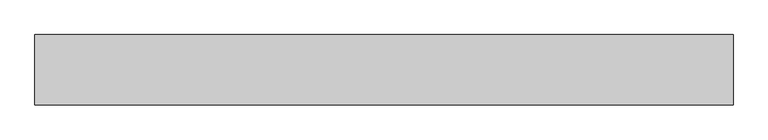
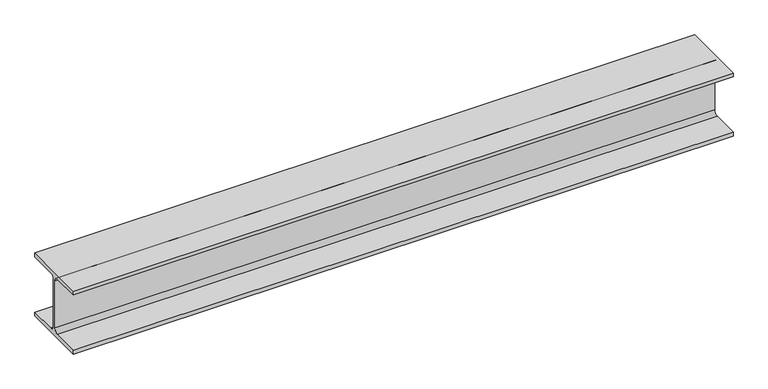
"""IFC4 building model written with IfcOpenShell, lengths in millimetres: beam geometry, 0912_Steel Framing_H-KSD3502 : H_SB_ASB_H-200x200x8x12."""

from ifc_helpers import new_model, si_unit, point, frame, frame_2d, origin, place, context, project, spatial, polyline, circle_curve, trimmed, segment, composite_curve, outline, extrude, source, transform, mapped, element, save


def beam_dd983640(model_context):
    return source(origin(), model_context, "Body", "SweptSolid", [
        extrude(outline(composite_curve([segment(polyline([(100.0, -88.0), (100.0, -100.0), (-100.0, -100.0), (-100.0, -88.0), (-17.0, -88.0)]), True, "CONTINUOUS"), segment(trimmed(circle_curve(frame_2d((-17.0, -75.0)), 13.0), [point((-17.0, -88.0))], [point((-4.0, -75.0))], True, "CARTESIAN"), True, "CONTINUOUS"), segment(polyline([(-4.0, -75.0), (-4.0, 75.0)]), True, "CONTINUOUS"), segment(trimmed(circle_curve(frame_2d((-17.0, 75.0)), 13.0), [point((-4.0, 75.0))], [point((-17.0, 88.0))], True, "CARTESIAN"), True, "CONTINUOUS"), segment(polyline([(-17.0, 88.0), (-100.0, 88.0), (-100.0, 100.0), (100.0, 100.0), (100.0, 88.0), (17.0, 88.0)]), True, "CONTINUOUS"), segment(trimmed(circle_curve(frame_2d((17.0, 75.0)), 13.0), [point((17.0, 88.0))], [point((4.0, 75.0))], True, "CARTESIAN"), True, "CONTINUOUS"), segment(polyline([(4.0, 75.0), (4.0, -75.0)]), True, "CONTINUOUS"), segment(trimmed(circle_curve(frame_2d((17.0, -75.0)), 13.0), [point((4.0, -75.0))], [point((17.0, -88.0))], True, "CARTESIAN"), True, "CONTINUOUS"), segment(polyline([(17.0, -88.0), (100.0, -88.0)]), True, "CONTINUOUS")], self_intersect=False)), frame((-1040.0605605, 0.0, 0.0), z_axis=(1.0, 0.0, 0.0), x_axis=(0.0, 1.0, 0.0)), (0.0, 0.0, 1.0), 1981.2854342),
    ])


if __name__ == "__main__":
    model = new_model("IFC4")
    model_context = context("Model", 3, world=origin())
    ifc_project = project(units=[si_unit("LENGTHUNIT", "METRE", prefix="MILLI")], contexts=[model_context])
    site = spatial("IfcSite", under=ifc_project)
    building = spatial("IfcBuilding", under=site)
    placement = place(None, origin())
    beam_shape = beam_dd983640(model_context)
    element("IfcBeam", 1, ObjectType="0912_Steel Framing_H-KSD3502 : H_SB_ASB_H-200x200x8x12", at=placement, inside=building, context=model_context, shape_type="MappedRepresentation", body=[
        mapped(beam_shape, transform((0.0, 0.0, 0.0), x_axis=(1.0, 0.0, 0.0), y_axis=(0.0, 1.0, 0.0), z_axis=(0.0, 0.0, 1.0))),
    ])
    save(model, "model.ifc")

# Revit data of these elements
# Type "0912_Steel Framing_H-KSD3502 : H_SB_ASB_H-200x200x8x12"
#   H_WM Code_1 = "S01AA002-00001 | Main Steel Structure Fabrication Work | Shelter/Building | Medium Steel - Standard (90KG/M>Weight≥30KG/M) | Material: (   )"
#   H_WM Code_2 = "S03AA028-00001 | Main Steel Structure Erection Work | Shelter/Building | Medium Steel (90KG/M>Weight≥30KG/M) | Material: (   )"
#   H_WM Code_3 = "S01AA010-00001 | Main Steel Structure Fabrication Work | Shelter/Building | Steel Painting/Coating | for Non-Fireproofed Steel Surface, Surface Preparation, Primer, Second & Final Coat | Material: (   )"
#   H_Q'ty Cal Type Tag = "SB-Q2"
#   Width = 20.0 cm
#   Web Thickness = 0.8 cm
#   Web Fillet = 1.3 cm
#   Warping Constant = 141000.0 cm⁶
#   W = 0
#   Torsional Moment of Inertia = 26.2485 cm⁴
#   Section Area = 63.53 cm²
#   Plastic Modulus weak axis = 244.0 cm³
#   Plastic Modulus strong axis = 525.0 cm³
#   Perimeter = 1.16 m²/m
#   Nominal Weight = 49.90 kgf/m
#   Moment of Inertia weak axis = 1600.00 cm⁴
#   Moment of Inertia strong axis = 4720.00 cm⁴
#   Height = 20.0 cm
#   Flange Thickness = 1.2 cm
#   Elastic Modulus weak axis = 160.0 cm³
#   Elastic Modulus strong axis = 472.0 cm³
#   Centroid Vertical = 10.0 cm
#   Centroid Horizontal = 10.0 cm
#   Ix = 47200000
#   Length [instance default] = 1.5240 m
#   Zx = 525000
#   b = 0.2000 m
#   h = 0.2000 m
#   r = 0.0130 m
#   s = 0.0080 m
#   t = 0.0120 m
#   A = 0.006353 m²
#   Structural Material [instance default] = Steel, 45-345
#   Assembly Code = ""
# Element 1 (IfcBeam, "0912_Steel Framing_H-KSD3502 : H_SB_ASB_H-200x200x8x12")
#   Structural Material = none
# Materials
#   "Steel, 45-345": class "Metal", colour RGB 189 187 185, transparency 0, Description = "Steel 345 MPa", Cost = 0
